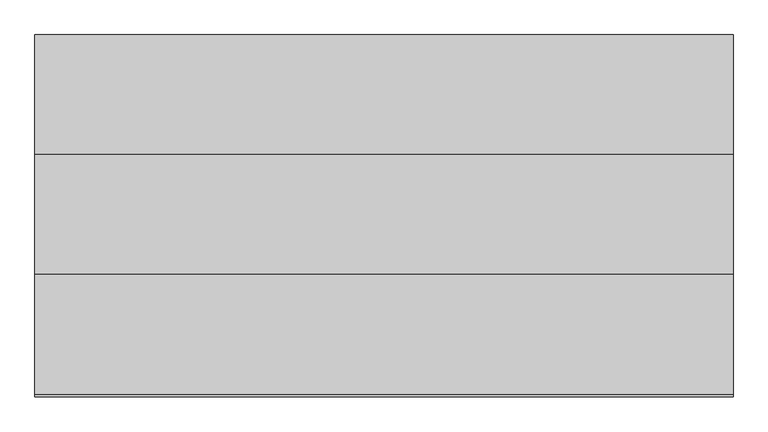
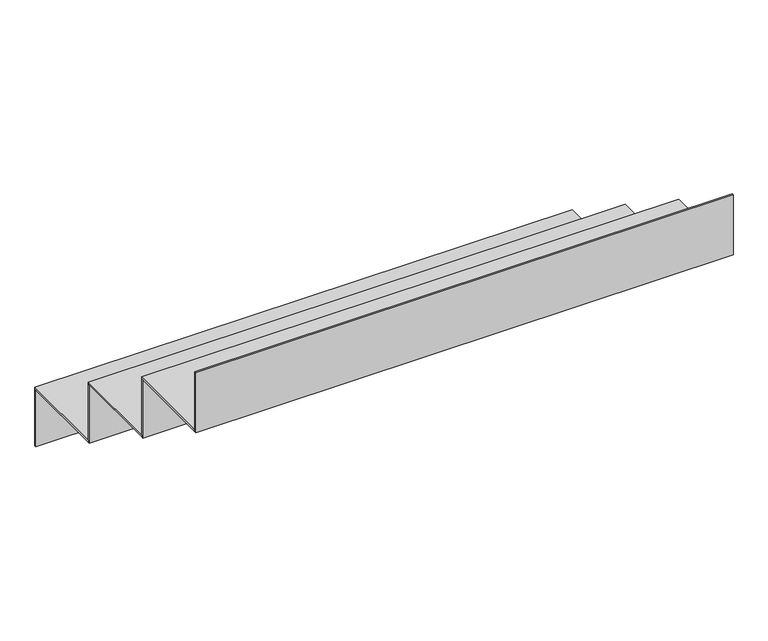
"""IFC4 building model written with IfcOpenShell, lengths in millimetres: stair flight geometry."""

from ifc_helpers import new_model, si_unit, frame, origin, place, context, project, spatial, polyline, outline, extrude, source, transform, mapped, element, save


def stair_flight_4d69585d(model_context):
    return source(origin(), model_context, "Body", "SweptSolid", [
        extrude(outline(polyline([(52905.0, -6206.0), (52905.0, -6200.0), (54650.0, -6200.0), (54650.0, -6206.0), (52905.0, -6206.0)])), frame((0.0, 0.0, 20000.0), z_axis=(0.0, 0.0, 1.0), x_axis=(1.0, 0.0, 0.0)), (0.0, 0.0, 1.0), 194.0),
        extrude(outline(polyline([(54650.0, -6500.0), (52905.0, -6500.0), (52905.0, -6200.0), (54650.0, -6200.0), (54650.0, -6500.0)])), frame((0.0, 0.0, 20194.0), z_axis=(0.0, 0.0, 1.0), x_axis=(1.0, 0.0, 0.0)), (0.0, 0.0, 1.0), 6.0),
        extrude(outline(polyline([(52905.0, -6506.0), (52905.0, -6500.0), (54650.0, -6500.0), (54650.0, -6506.0), (52905.0, -6506.0)])), frame((0.0, 0.0, 20194.0), z_axis=(0.0, 0.0, 1.0), x_axis=(1.0, 0.0, 0.0)), (0.0, 0.0, 1.0), 200.0),
        extrude(outline(polyline([(54650.0, -6800.0), (52905.0, -6800.0), (52905.0, -6500.0), (54650.0, -6500.0), (54650.0, -6800.0)])), frame((0.0, 0.0, 20394.0), z_axis=(0.0, 0.0, 1.0), x_axis=(1.0, 0.0, 0.0)), (0.0, 0.0, 1.0), 6.0),
        extrude(outline(polyline([(52905.0, -6806.0), (52905.0, -6800.0), (54650.0, -6800.0), (54650.0, -6806.0), (52905.0, -6806.0)])), frame((0.0, 0.0, 20394.0), z_axis=(0.0, 0.0, 1.0), x_axis=(1.0, 0.0, 0.0)), (0.0, 0.0, 1.0), 200.0),
        extrude(outline(polyline([(54650.0, -7100.0), (52905.0, -7100.0), (52905.0, -6800.0), (54650.0, -6800.0), (54650.0, -7100.0)])), frame((0.0, 0.0, 20594.0), z_axis=(0.0, 0.0, 1.0), x_axis=(1.0, 0.0, 0.0)), (0.0, 0.0, 1.0), 6.0),
        extrude(outline(polyline([(52905.0, -7106.0), (52905.0, -7100.0), (54650.0, -7100.0), (54650.0, -7106.0), (52905.0, -7106.0)])), frame((0.0, 0.0, 20594.0), z_axis=(0.0, 0.0, 1.0), x_axis=(1.0, 0.0, 0.0)), (0.0, 0.0, 1.0), 206.0),
    ])


if __name__ == "__main__":
    model = new_model("IFC4")
    model_context = context("Model", 3, world=origin())
    ifc_project = project(units=[si_unit("LENGTHUNIT", "METRE", prefix="MILLI")], contexts=[model_context])
    site = spatial("IfcSite", under=ifc_project)
    building = spatial("IfcBuilding", under=site)
    placement = place(None, origin())
    stair_flight_shape = stair_flight_4d69585d(model_context)
    element("IfcStairFlight", 1, at=placement, inside=building, context=model_context, shape_type="MappedRepresentation", body=[
        mapped(stair_flight_shape, transform((0.0, 0.0, 0.0), x_axis=(1.0, 0.0, 0.0), y_axis=(0.0, 1.0, 0.0), z_axis=(0.0, 0.0, 1.0))),
    ])
    save(model, "model.ifc")

# Revit data of these elements
# Element 1 (IfcStairFlight)
#   Materials on its faces: "Checkered Plate"
# Materials
#   "Checkered Plate": class "Metal", colour RGB 84 83 81, transparency 0, Description = "Steel, mill finish", Cost = 0
